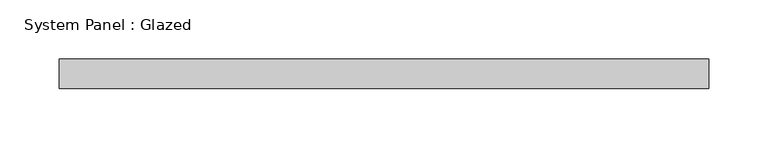
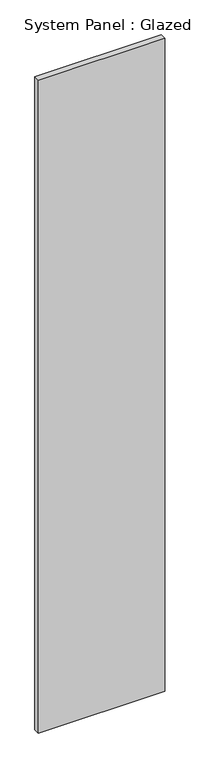
"""IFC4 building model written with IfcOpenShell, lengths in millimetres: plate geometry, System Panel : Glazed."""

from ifc_helpers import new_model, si_unit, origin, origin_with_axes, place, context, project, spatial, polyline, outline, extrude, source, transform, mapped, element, save


def system_panel_glazed_a36a1bad(model_context):
    return source(origin(), model_context, "Body", "SweptSolid", [
        extrude(outline(polyline([(274.9999998, 24.5), (-274.9999998, 24.5), (-274.9999998, 49.5), (274.9999998, 49.5), (274.9999998, 24.5)])), origin_with_axes(), (0.0, 0.0, 1.0), 3000.0),
    ])


if __name__ == "__main__":
    model = new_model("IFC4")
    model_context = context("Model", 3, world=origin())
    ifc_project = project(units=[si_unit("LENGTHUNIT", "METRE", prefix="MILLI")], contexts=[model_context])
    site = spatial("IfcSite", under=ifc_project)
    building = spatial("IfcBuilding", under=site)
    placement = place(None, origin())
    system_panel_glazed_shape = system_panel_glazed_a36a1bad(model_context)
    element("IfcPlate", 1, ObjectType="System Panel : Glazed", at=placement, inside=building, context=model_context, shape_type="MappedRepresentation", body=[
        mapped(system_panel_glazed_shape, transform((0.0, 0.0, 0.0), x_axis=(1.0, 0.0, 0.0), y_axis=(0.0, 1.0, 0.0), z_axis=(0.0, 0.0, 1.0))),
    ])
    save(model, "model.ifc")

# Revit data of these elements
# Type "System Panel : Glazed"
#   Construction Type Id = "GSP4R"
#   Analytic Construction = "1/8 in Pilkington single glazing"
#   Visual Light Transmittance = 0.9
#   Solar Heat Gain Coefficient = 0.86
#   Heat Transfer Coefficient (U) = 6.7069 W/(m²·K)
#   Define Thermal Properties by = 1
# Element 1 (IfcPlate, "System Panel : Glazed")
#   Materials on its faces: "Glass"
# Materials
#   "Glass": class "Glass", colour RGB 0 128 192, transparency 0.9, Description = "Soda Lime Glass", Cost = 0
